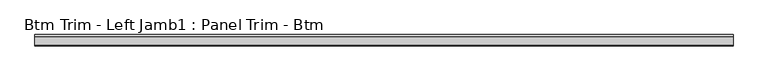
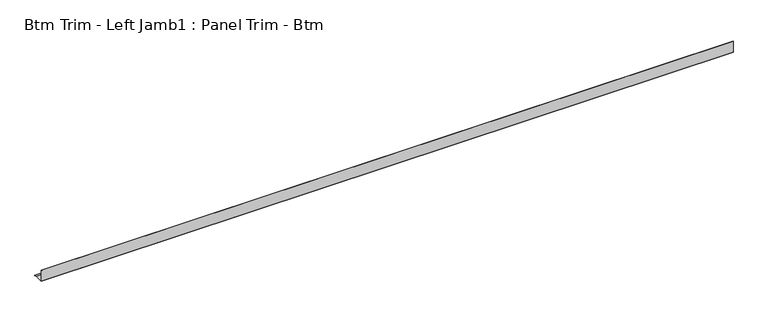
"""IFC4 building model written with IfcOpenShell, lengths in millimetres: proxy geometry, Btm Trim - Left Jamb1 : Panel Trim - Btm."""

import ifcopenshell
import ifcopenshell.guid

model = None  # the IFC model being written
_history = None  # IfcOwnerHistory: only IFC2X3 demands one
_inside = {}  # id of a spatial element -> (the spatial element, [elements in it])
_under = {}  # id of a project, library or spatial element -> (it, [spatial elements below it])
_declared = {}  # id of a project -> (the project, [libraries it declares])
_typed = {}  # id of a type object -> (the type object, [elements of that type])
_made_of = {}  # id of a material, layer set ... -> (it, [elements and type objects made of it])


def new_model(schema):
    """Start an empty IFC model of exactly this schema.

    Asked for "IFC4X3", IfcOpenShell would pick the latest addendum, in which some entities
    have other attributes; the version numbers below select the first issue.
    IFC2X3 requires an IfcOwnerHistory on every rooted entity: one is made here for all.
    """
    global model, _history
    if schema == "IFC4X3":
        model = ifcopenshell.file(schema_version=(4, 3, 0, 0))
    else:
        model = ifcopenshell.file(schema=schema)
    _inside.clear()
    _under.clear()
    _declared.clear()
    _typed.clear()
    _made_of.clear()
    _history = None
    if model.schema == "IFC2X3":
        org = make("IfcOrganization", Name="unknown")
        user = make(
            "IfcPersonAndOrganization",
            ThePerson=make("IfcPerson", FamilyName="unknown"),
            TheOrganization=org,
        )
        app = make(
            "IfcApplication",
            ApplicationDeveloper=org,
            Version="unknown",
            ApplicationFullName="unknown",
            ApplicationIdentifier="unknown",
        )
        _history = make(
            "IfcOwnerHistory",
            OwningUser=user,
            OwningApplication=app,
            ChangeAction="ADDED",
            CreationDate=0,
        )
    return model


def make(cls, **values):
    """One entity of the class cls with the attributes given. An attribute that is None is left unset."""
    return model.create_entity(
        cls, **{name: value for name, value in values.items() if value is not None}
    )


def rooted(cls, **values):
    """An entity with a GlobalId (a new one), such as an element, a storey or a relation."""
    return make(cls, GlobalId=ifcopenshell.guid.new(), OwnerHistory=_history, **values)


def si_unit(unit_type, name, prefix=None):
    """IfcSIUnit, for example si_unit("LENGTHUNIT", "METRE", prefix="MILLI")."""
    return make("IfcSIUnit", UnitType=unit_type, Prefix=prefix, Name=name)


def assignment(units):
    """IfcUnitAssignment: the units of a project."""
    return None if units is None else make("IfcUnitAssignment", Units=units)


def point(xyz):
    """IfcCartesianPoint."""
    return None if xyz is None else make("IfcCartesianPoint", Coordinates=xyz)


def direction(xyz):
    """IfcDirection."""
    return None if xyz is None else make("IfcDirection", DirectionRatios=xyz)


def frame(location, z_axis=None, x_axis=None):
    """IfcAxis2Placement3D, a coordinate frame: its origin and axes. An axis left out is left unset."""
    return make(
        "IfcAxis2Placement3D",
        Location=point(location),
        Axis=direction(z_axis),
        RefDirection=direction(x_axis),
    )


def origin():
    """The frame at (0, 0, 0) with its axes left unset."""
    return frame((0.0, 0.0, 0.0))


def place(relative_to, where):
    """IfcLocalPlacement: puts the frame where relative to a parent placement (None: the world)."""
    return make(
        "IfcLocalPlacement", PlacementRelTo=relative_to, RelativePlacement=where
    )


def context(
    kind, dimensions, precision=None, world=None, true_north=None, identifier=None
):
    """IfcGeometricRepresentationContext, for example the 3D "Model" context."""
    return make(
        "IfcGeometricRepresentationContext",
        ContextIdentifier=identifier,
        ContextType=kind,
        CoordinateSpaceDimension=dimensions,
        Precision=precision,
        WorldCoordinateSystem=world,
        TrueNorth=true_north,
    )


def project(units=None, contexts=None):
    """IfcProject with its units and contexts."""
    return rooted(
        "IfcProject",
        Name="project",
        RepresentationContexts=contexts,
        UnitsInContext=assignment(units),
    )


def spatial(cls, under=None, at=None, **own):
    """A site, building, storey or space (cls), placed at a placement, below another one or the project."""
    s = rooted(cls, ObjectPlacement=at, **own)
    if under is not None:
        _under.setdefault(under.id(), (under, []))[1].append(s)
    return s


def polyline(points):
    """IfcPolyline through the points."""
    return make("IfcPolyline", Points=[point(p) for p in points])


def outline(outer, holes=None, kind="AREA"):
    """IfcArbitraryClosedProfileDef: a profile drawn as a closed curve; with holes, ...WithVoids."""
    if holes is None:
        return make("IfcArbitraryClosedProfileDef", ProfileType=kind, OuterCurve=outer)
    return make(
        "IfcArbitraryProfileDefWithVoids",
        ProfileType=kind,
        OuterCurve=outer,
        InnerCurves=holes,
    )


def extrude(swept, where, along, depth):
    """IfcExtrudedAreaSolid: the profile swept, set in the frame where, extruded along a direction by depth."""
    return make(
        "IfcExtrudedAreaSolid",
        SweptArea=swept,
        Position=where,
        ExtrudedDirection=direction(along),
        Depth=depth,
    )


def shape(context_of_items, identifier, shape_type, items):
    """IfcShapeRepresentation: the items that make up one representation, for example the "Body"."""
    return make(
        "IfcShapeRepresentation",
        ContextOfItems=context_of_items,
        RepresentationIdentifier=identifier,
        RepresentationType=shape_type,
        Items=items,
    )


def source(mapping_origin, context_of_items, identifier, shape_type, items):
    """IfcRepresentationMap: a shape defined once, which mapped items show again and again."""
    return make(
        "IfcRepresentationMap",
        MappingOrigin=mapping_origin,
        MappedRepresentation=shape(context_of_items, identifier, shape_type, items),
    )


def transform(
    local_origin,
    x_axis=None,
    y_axis=None,
    z_axis=None,
    scale=None,
    scale2=None,
    scale3=None,
    uniform=True,
):
    """IfcCartesianTransformationOperator3D, or its non-uniform kind. x_axis, y_axis, z_axis: its Axis1, 2, 3."""
    if uniform:
        return make(
            "IfcCartesianTransformationOperator3D",
            Axis1=direction(x_axis),
            Axis2=direction(y_axis),
            LocalOrigin=point(local_origin),
            Scale=scale,
            Axis3=direction(z_axis),
        )
    return make(
        "IfcCartesianTransformationOperator3DnonUniform",
        Axis1=direction(x_axis),
        Axis2=direction(y_axis),
        LocalOrigin=point(local_origin),
        Scale=scale,
        Axis3=direction(z_axis),
        Scale2=scale2,
        Scale3=scale3,
    )


def mapped(mapping_source, mapping_target):
    """IfcMappedItem: shows the shape of a source again, moved by a transform."""
    return make(
        "IfcMappedItem", MappingSource=mapping_source, MappingTarget=mapping_target
    )


def made_of(thing, what):
    """Note that an element or type object is made of a material, layer set ...; save() writes the relation."""
    if what is not None:
        _made_of.setdefault(what.id(), (what, []))[1].append(thing)
    return thing


def element(
    cls,
    number,
    at=None,
    inside=None,
    cuts=None,
    type_object=None,
    material=None,
    context=None,
    identifier="Body",
    shape_type=None,
    held_by="IfcProductDefinitionShape",
    body=None,
    shapes=None,
    **own,
):
    """One element of the class cls, such as IfcWall. Its Tag is "e" and its number.

    at: its placement. inside: the storey or other place that contains it. cuts: it is an
    opening in that element (IfcRelVoidsElement). A single representation is given by context,
    identifier, shape_type and body (its items); several are given by shapes. held_by: the class
    of the entity that holds the representations. save() writes the other relations.
    """
    e = rooted(cls, Tag="e%d" % number, ObjectPlacement=at, **own)
    if body is not None:
        shapes = [shape(context, identifier, shape_type, body)]
    if shapes is not None:
        e.Representation = make(held_by, Representations=shapes)
    if inside is not None:
        _inside.setdefault(inside.id(), (inside, []))[1].append(e)
    if cuts is not None:
        rooted(
            "IfcRelVoidsElement", RelatingBuildingElement=cuts, RelatedOpeningElement=e
        )
    if type_object is not None:
        _typed.setdefault(type_object.id(), (type_object, []))[1].append(e)
    return made_of(e, material)


def aggregate(whole, parts):
    """IfcRelAggregates: a whole, such as a stair, and the parts it consists of."""
    return rooted("IfcRelAggregates", RelatingObject=whole, RelatedObjects=parts)


def save(model, path):
    """Write the relations noted so far, then the file.

    IfcRelAggregates (storeys below a building ...), IfcRelContainedInSpatialStructure (elements
    in a storey), IfcRelDefinesByType, IfcRelAssociatesMaterial and IfcRelDeclares: one each for
    every whole, place, type object, material and project.
    """
    for whole, parts in _under.values():
        aggregate(whole, parts)
    for where, things in _inside.values():
        rooted(
            "IfcRelContainedInSpatialStructure",
            RelatedElements=things,
            RelatingStructure=where,
        )
    for kind, things in _typed.values():
        rooted("IfcRelDefinesByType", RelatedObjects=things, RelatingType=kind)
    for what, things in _made_of.values():
        rooted("IfcRelAssociatesMaterial", RelatedObjects=things, RelatingMaterial=what)
    for by, libraries in _declared.values():
        rooted("IfcRelDeclares", RelatingContext=by, RelatedDefinitions=libraries)
    model.write(path)


def btm_trim_left_jamb1_panel_trim_btm_b9c60ca2(model_context):
    return source(origin(), model_context, "Body", "SweptSolid", [
        extrude(outline(polyline([(-531600.2244849, 0.79375), (-531590.923103, -1.6985478), (-531591.1285406, -2.4652514), (-531600.3289841, 0.0), (-531640.0037841, 0.0), (-531640.0037841, 51.59375), (-531639.2163841, 51.59375), (-531639.2163841, 0.79375), (-531600.2244849, 0.79375)])), frame((587327.7998239, 0.0, 0.0), z_axis=(1.0, 0.0, 0.0), x_axis=(0.0, 1.0, 0.0)), (0.0, 0.0, 1.0), 3063.2733375),
    ])


if __name__ == "__main__":
    model = new_model("IFC4")
    model_context = context("Model", 3, world=origin())
    ifc_project = project(units=[si_unit("LENGTHUNIT", "METRE", prefix="MILLI")], contexts=[model_context])
    site = spatial("IfcSite", under=ifc_project)
    building = spatial("IfcBuilding", under=site)
    placement = place(None, origin())
    btm_trim_left_jamb1_panel_trim_btm_shape = btm_trim_left_jamb1_panel_trim_btm_b9c60ca2(model_context)
    element("IfcBuildingElementProxy", 1, Name="Btm Trim - Left Jamb1 : Panel Trim - Btm", ObjectType="Btm Trim - Left Jamb1 : Panel Trim - Btm", at=placement, inside=building, context=model_context, shape_type="MappedRepresentation", body=[
        mapped(btm_trim_left_jamb1_panel_trim_btm_shape, transform((0.0, 0.0, 0.0), x_axis=(1.0, 0.0, 0.0), y_axis=(0.0, 1.0, 0.0), z_axis=(0.0, 0.0, 1.0))),
    ])
    save(model, "model.ifc")

# Revit data of these elements
# Element 1 (IfcBuildingElementProxy, "Btm Trim - Left Jamb1 : Panel Trim - Btm")
#   Materials on its faces: "BASE TRIM BY MTL PANEL MFR."
# Materials
#   "BASE TRIM BY MTL PANEL MFR.": class "Generic", colour RGB 239 242 240, transparency 0, Cost = 0
